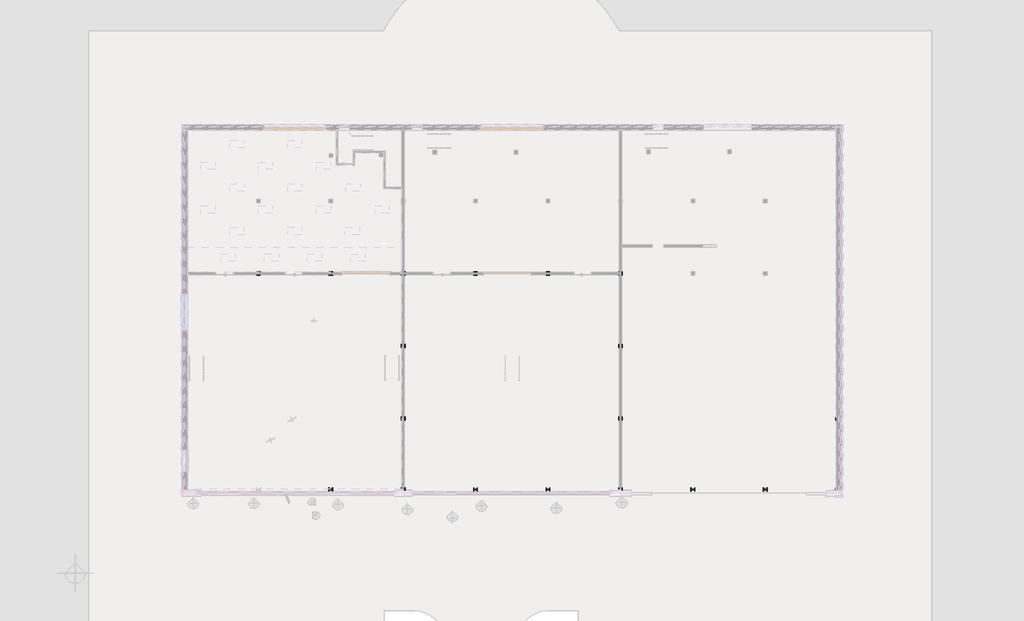
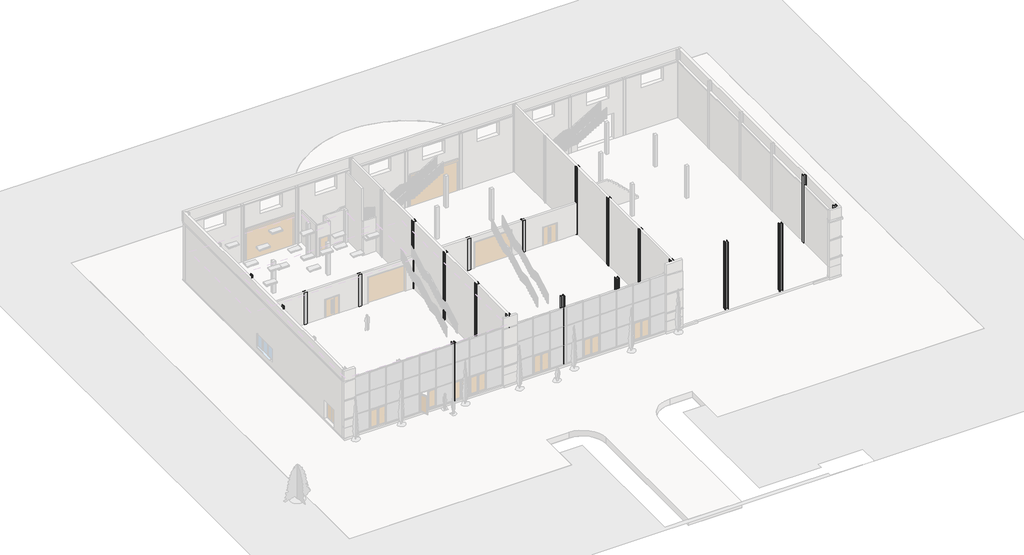
# One storey, part 5 of 13: 21 columns, 21 slabs, 8 footings.
# Revit data of these elements (continued)
# Grids (mm) (continued)
#   "9": line (40860.445, -23439.181) -> (40860.445, 8028.559)
#   "D": line (-7587.705, -11058.762) -> (47341.061, -11058.762)
#   "E": line (-7587.705, -17058.762) -> (47341.061, -17058.762)
#   "10": line (46860.445, -23439.181) -> (46860.445, 8028.559)
#   "F": line (-7587.705, -22948.762) -> (47341.061, -22948.762)
# Type "Concrete Square : 300 x 300mm"
#   Keynote = "E"
#   b = 300 mm
#   Structural Material [instance default] = Concrete - Cast-in-Place Concrete
# Type "UC-Universal Column-Column : 305x305x97UC"
#   Keynote = "G10"
#   Nominal h = ""
#   W = 0
#   Ix = 0
#   M = 96.9
#   Zx = 0
#   b = 305.3 mm
#   h = 307.9 mm
#   r = 15.2 mm
#   s = 9.9 mm
#   t = 15.4 mm
#   A = 123 m²
#   Structural Material [instance default] = Steel, 45-345
#   Assembly Code = ""
# Type "Pad Foundation-Rectangular : 1000x1000x500"
#   Reinforcement Specs [instance default] = ""
#   Pad Type = "P1"
#   Mesh [instance default] = ""
#   Concrete Grade [instance default] = ""
#   Volume = 0.50 m³
#   Pad Width = 1000 mm
#   Pad Length = 1000 mm
#   Pad Depth = 500 mm
#   Structural Material [instance default] = Concrete - Cast-in-Place Concrete
# Elements 1, 2, 3, 4 (IfcColumn, "Concrete Square : 300 x 300mm")
#   Comments = ""
#   Phase Created = New Construction
#   Materials on its faces: "Concrete - Cast-in-Place Concrete"
# Elements 5, 6, 7, 8, 9, 10, 11, 12, 13, 14, 15, 16, 17, 18, 19, 20, 21 (IfcColumn, "UC-Universal Column-Column : 305x305x97UC")
#   Comments = ""
#   Structural Material = Steel, 45-345
#   Phase Created = New Construction
#   Materials on its faces: "Steel, 45-345"
# Elements 22, 23, 24, 25, 26, 27 (IfcFooting, "Wall Foundation - Commercial 1300 x 450")
#   Phase Created = New Construction
#   Materials on its faces: "Concrete, Cast In Situ"
# Elements 28, 29 (IfcFooting, "Wall Foundation - Commercial 1300 x 450")
#   Comments = ""
#   Phase Created = New Construction
#   Materials on its faces: "Concrete, Cast In Situ"
# Elements 30, 31, 32, 33, 34, 35, 36, 37, 38, 39, 40, 41, 42, 43, 44, 45, 46, 47, 48, 49, 50 (IfcSlab, "Pad Foundation-Rectangular : 1000x1000x500")
#   Comments = ""
#   Reinforcement Specs = ""
#   Mesh = ""
#   Concrete Grade = ""
#   Structural Material = Concrete - Cast-in-Place Concrete
#   Phase Created = New Construction
#   Materials on its faces: "Concrete - Cast-in-Place Concrete"
# Materials
#   "Concrete - Cast-in-Place Concrete": class "Concrete", colour RGB 192 192 192, transparency 0
#   "Steel, 45-345": class "Metal", colour RGB 247 247 247, transparency 0, Description = "Steel 345 MPa", Cost = 0
#   "Concrete, Cast In Situ": class "Concrete", colour RGB 192 192 192, transparency 0, Description = "physical material", Cost = 0
# Room at (2534.039, 34.316) mm, phase "New Construction", upper level "L0 - Ground Floor (Shadows On)", upper offset 4000 mm, lower offset 0 mm
#   Number = "1"
#   Name = "Room"
# Room at (2390.683, -14731.423) mm, phase "New Construction", upper level "L0 - Ground Floor (Shadows On)", upper offset 4000 mm, lower offset 0 mm
#   Number = "2"
#   Name = "Room"
